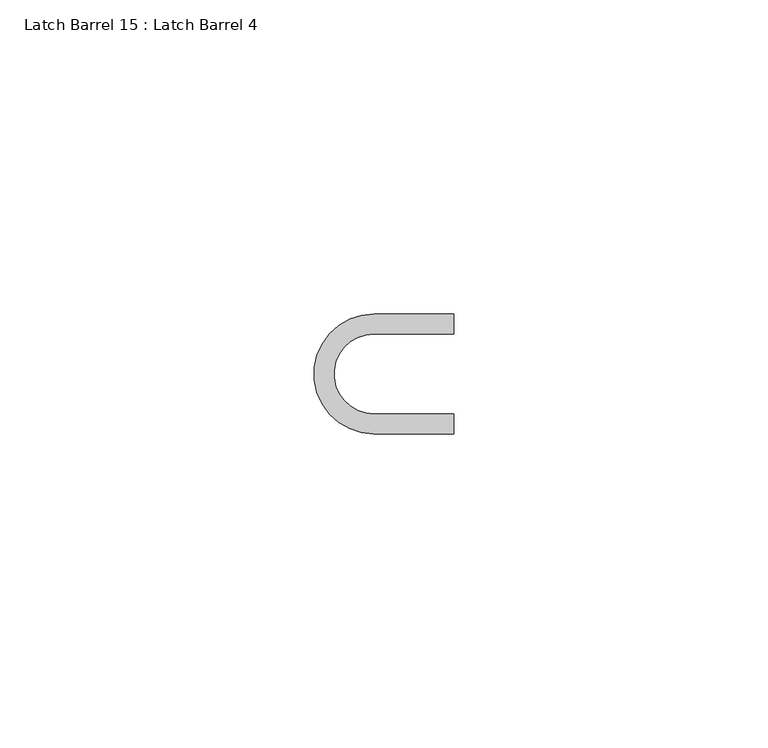
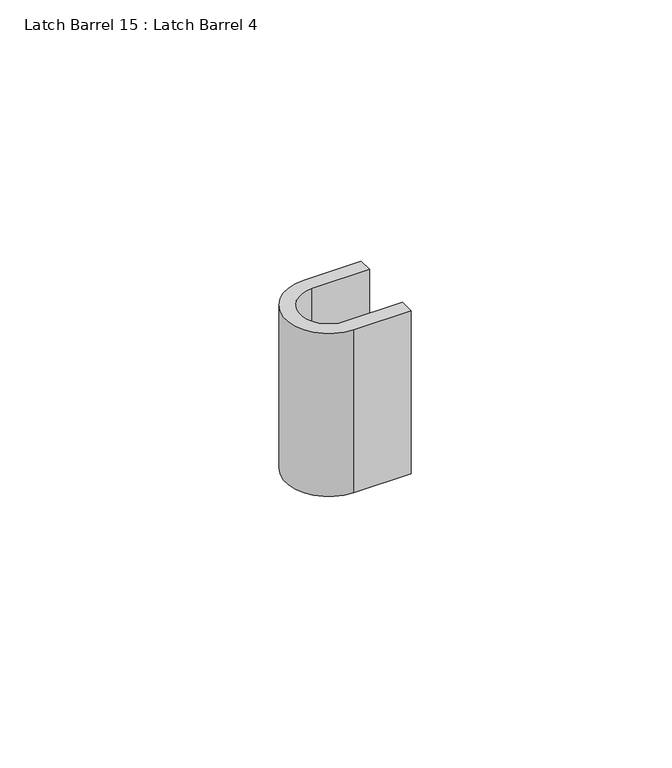
"""IFC4 building model written with IfcOpenShell, lengths in millimetres: proxy geometry, Latch Barrel 15 : Latch Barrel 4."""

from ifc_helpers import new_model, si_unit, point, frame, frame_2d, origin, place, context, project, spatial, polyline, circle_curve, trimmed, segment, composite_curve, outline, extrude, source, transform, mapped, element, save


def latch_barrel_15_latch_barrel_4_f16c52b4(model_context):
    return source(origin(), model_context, "Body", "SweptSolid", [
        extrude(outline(composite_curve([segment(trimmed(circle_curve(frame_2d((587309.5435739, -532839.3663841)), 6.35), [point((587309.5435739, -532833.0163841))], [point((587309.5435739, -532845.7163841))], True, "CARTESIAN"), True, "CONTINUOUS"), segment(polyline([(587309.5435739, -532845.7163841), (587322.2435739, -532845.7163841), (587322.2435739, -532848.8913841), (587309.5435739, -532848.8913841)]), True, "CONTINUOUS"), segment(trimmed(circle_curve(frame_2d((587309.5435739, -532839.3663841)), 9.525), [point((587309.5435739, -532848.8913841))], [point((587309.5435739, -532829.8413841))], False, "CARTESIAN"), True, "CONTINUOUS"), segment(polyline([(587309.5435739, -532829.8413841), (587322.2435739, -532829.8413841), (587322.2435739, -532833.0163841), (587309.5435739, -532833.0163841)]), True, "CONTINUOUS")], self_intersect=False)), frame((0.0, 0.0, 241.3), z_axis=(0.0, 0.0, 1.0), x_axis=(1.0, 0.0, 0.0)), (0.0, 0.0, 1.0), 38.1),
    ])


if __name__ == "__main__":
    model = new_model("IFC4")
    model_context = context("Model", 3, world=origin())
    ifc_project = project(units=[si_unit("LENGTHUNIT", "METRE", prefix="MILLI")], contexts=[model_context])
    site = spatial("IfcSite", under=ifc_project)
    building = spatial("IfcBuilding", under=site)
    placement = place(None, origin())
    latch_barrel_15_latch_barrel_4_shape = latch_barrel_15_latch_barrel_4_f16c52b4(model_context)
    element("IfcBuildingElementProxy", 1, Name="Latch Barrel 15 : Latch Barrel 4", ObjectType="Latch Barrel 15 : Latch Barrel 4", at=placement, inside=building, context=model_context, shape_type="MappedRepresentation", body=[
        mapped(latch_barrel_15_latch_barrel_4_shape, transform((0.0, 0.0, 0.0), x_axis=(1.0, 0.0, 0.0), y_axis=(0.0, 1.0, 0.0), z_axis=(0.0, 0.0, 1.0))),
    ])
    save(model, "model.ifc")

# Revit data of these elements
# Element 1 (IfcBuildingElementProxy, "Latch Barrel 15 : Latch Barrel 4")
#   Materials on its faces: "GALV. SLIDE BOLT"
# Materials
#   "GALV. SLIDE BOLT": class "Metal", colour RGB 189 187 185, transparency 0, Description = "Carbon steel", Cost = 0
